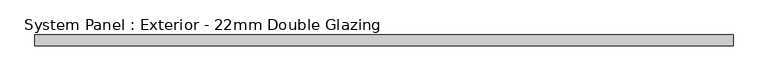
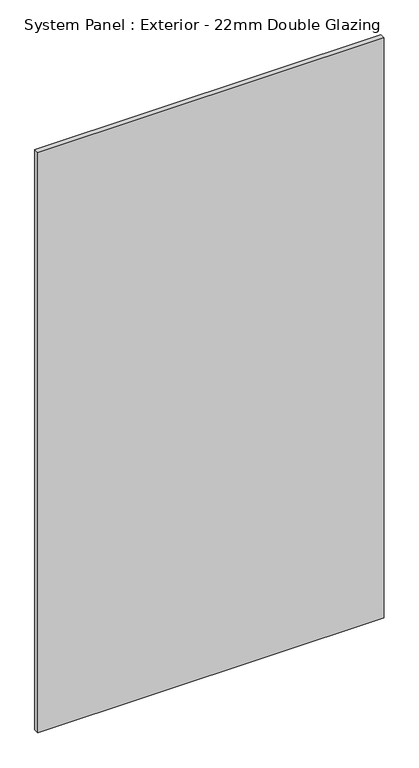
"""IFC4 building model written with IfcOpenShell, lengths in millimetres: plate geometry, System Panel : Exterior - 22mm Double Glazing."""

from ifc_helpers import new_model, si_unit, origin, origin_with_axes, place, context, project, spatial, polyline, outline, extrude, source, transform, mapped, element, save


def system_panel_exterior_22mm_double_glazing_2405d1dc(model_context):
    return source(origin(), model_context, "Body", "SweptSolid", [
        extrude(outline(polyline([(712.5000001, 15.0), (-712.5000001, 15.0), (-712.5000001, 37.0), (712.5000001, 37.0), (712.5000001, 15.0)])), origin_with_axes(), (0.0, 0.0, 1.0), 2525.0),
    ])


if __name__ == "__main__":
    model = new_model("IFC4")
    model_context = context("Model", 3, world=origin())
    ifc_project = project(units=[si_unit("LENGTHUNIT", "METRE", prefix="MILLI")], contexts=[model_context])
    site = spatial("IfcSite", under=ifc_project)
    building = spatial("IfcBuilding", under=site)
    placement = place(None, origin())
    system_panel_exterior_22mm_double_glazing_shape = system_panel_exterior_22mm_double_glazing_2405d1dc(model_context)
    element("IfcPlate", 1, ObjectType="System Panel : Exterior - 22mm Double Glazing", at=placement, inside=building, context=model_context, shape_type="MappedRepresentation", body=[
        mapped(system_panel_exterior_22mm_double_glazing_shape, transform((0.0, 0.0, 0.0), x_axis=(1.0, 0.0, 0.0), y_axis=(0.0, 1.0, 0.0), z_axis=(0.0, 0.0, 1.0))),
    ])
    save(model, "model.ifc")

# Revit data of these elements
# Element 1 (IfcPlate, "System Panel : Exterior - 22mm Double Glazing")
#   Materials on its faces: "Glass"
# Materials
#   "Glass": class "Glass", colour RGB 180 200 255, transparency 0.75, Description = "Generisk glas", Cost = 0
